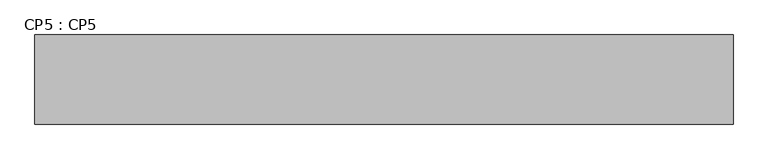
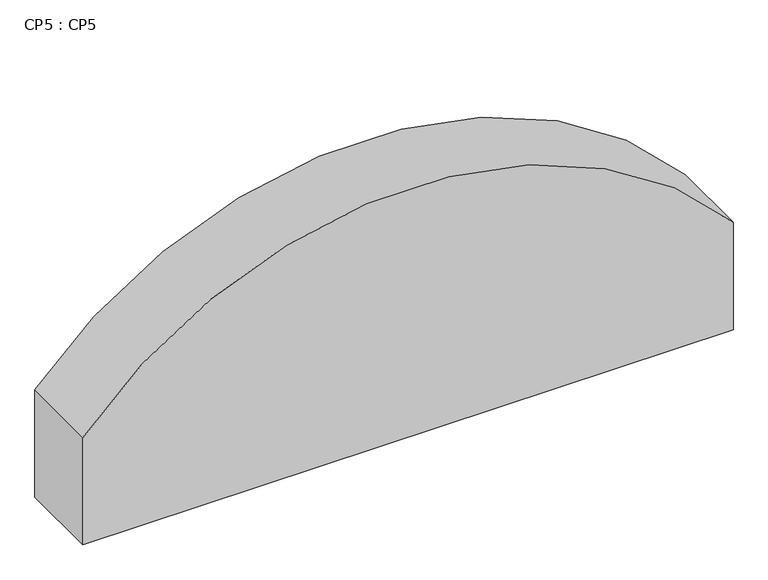
"""IFC4 building model written with IfcOpenShell, lengths in millimetres: beam geometry, CP5 : CP5."""

from ifc_helpers import new_model, si_unit, point, frame, frame_2d, origin, place, context, project, spatial, polyline, circle_curve, trimmed, segment, composite_curve, outline, extrude, source, transform, mapped, element, save


def cp5_cp5_4d0b3d9a(model_context):
    return source(origin(), model_context, "Body", "SweptSolid", [
        extrude(outline(composite_curve([segment(trimmed(circle_curve(frame_2d((12608.2612414, 27833.2245515)), 3093.4758497), [point((14620.0, 30183.2245515))], [point((14620.0, 25483.2245516))], False, "CARTESIAN"), True, "CONTINUOUS"), segment(polyline([(14620.0, 25483.2245516), (13800.0, 25483.2245516), (13800.0, 30183.2245515), (14620.0, 30183.2245515)]), True, "CONTINUOUS")], self_intersect=False)), frame((0.0, -100.2551788, 0.0), z_axis=(0.0, 1.0, 0.0), x_axis=(0.0, 0.0, 1.0)), (0.0, 0.0, 1.0), 599.9551778),
    ])


if __name__ == "__main__":
    model = new_model("IFC4")
    model_context = context("Model", 3, world=origin())
    ifc_project = project(units=[si_unit("LENGTHUNIT", "METRE", prefix="MILLI")], contexts=[model_context])
    site = spatial("IfcSite", under=ifc_project)
    building = spatial("IfcBuilding", under=site)
    placement = place(None, origin())
    cp5_cp5_shape = cp5_cp5_4d0b3d9a(model_context)
    element("IfcBeam", 1, ObjectType="CP5 : CP5", at=placement, inside=building, context=model_context, shape_type="MappedRepresentation", body=[
        mapped(cp5_cp5_shape, transform((0.0, 0.0, 0.0), x_axis=(1.0, 0.0, 0.0), y_axis=(0.0, 1.0, 0.0), z_axis=(0.0, 0.0, 1.0))),
    ])
    save(model, "model.ifc")
